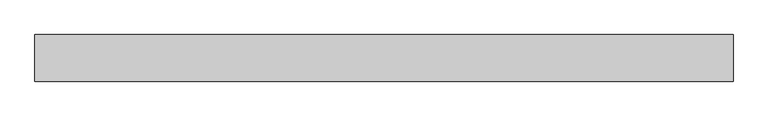
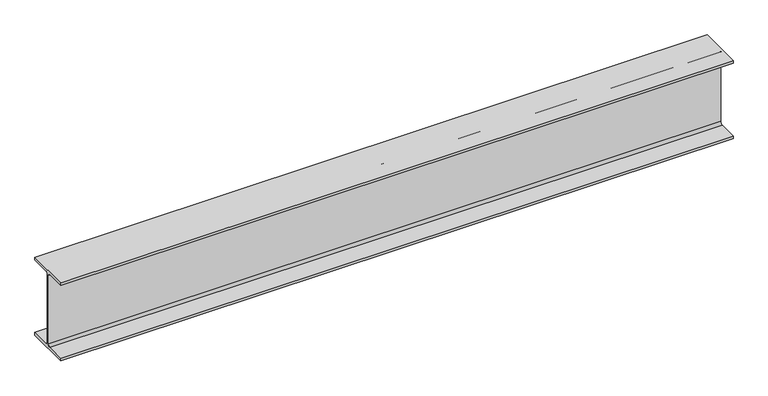
"""IFC4 building model written with IfcOpenShell, lengths in millimetres: beam geometry, Old_Steel Beam_H-KSD3502 : H_SB_ASB_H-350×175x7x11."""

from ifc_helpers import new_model, si_unit, point, frame, frame_2d, origin, place, context, project, spatial, polyline, circle_curve, trimmed, segment, composite_curve, outline, extrude, source, transform, mapped, element, save


def beam_1666eb2f(model_context):
    return source(origin(), model_context, "Body", "SweptSolid", [
        extrude(outline(composite_curve([segment(polyline([(82.5, -141.5), (82.5, -151.7), (-82.5, -151.7), (-82.5, -141.5), (-11.9, -141.5)]), True, "CONTINUOUS"), segment(trimmed(circle_curve(frame_2d((-11.9, -132.6)), 8.9), [point((-11.9, -141.5))], [point((-3.0, -132.6))], True, "CARTESIAN"), True, "CONTINUOUS"), segment(polyline([(-3.0, -132.6), (-3.0, 132.6)]), True, "CONTINUOUS"), segment(trimmed(circle_curve(frame_2d((-11.9, 132.6)), 8.9), [point((-3.0, 132.6))], [point((-11.9, 141.5))], True, "CARTESIAN"), True, "CONTINUOUS"), segment(polyline([(-11.9, 141.5), (-82.5, 141.5), (-82.5, 151.7), (82.5, 151.7), (82.5, 141.5), (11.9, 141.5)]), True, "CONTINUOUS"), segment(trimmed(circle_curve(frame_2d((11.9, 132.6)), 8.9), [point((11.9, 141.5))], [point((3.0, 132.6))], True, "CARTESIAN"), True, "CONTINUOUS"), segment(polyline([(3.0, 132.6), (3.0, -132.6)]), True, "CONTINUOUS"), segment(trimmed(circle_curve(frame_2d((11.9, -132.6)), 8.9), [point((3.0, -132.6))], [point((11.9, -141.5))], True, "CARTESIAN"), True, "CONTINUOUS"), segment(polyline([(11.9, -141.5), (82.5, -141.5)]), True, "CONTINUOUS")], self_intersect=False)), frame((-1175.6379608, 0.0, 0.0), z_axis=(1.0, 0.0, 0.0), x_axis=(0.0, 1.0, 0.0)), (0.0, 0.0, 1.0), 2471.4118659),
    ])


if __name__ == "__main__":
    model = new_model("IFC4")
    model_context = context("Model", 3, world=origin())
    ifc_project = project(units=[si_unit("LENGTHUNIT", "METRE", prefix="MILLI")], contexts=[model_context])
    site = spatial("IfcSite", under=ifc_project)
    building = spatial("IfcBuilding", under=site)
    placement = place(None, origin())
    beam_shape = beam_1666eb2f(model_context)
    element("IfcBeam", 1, ObjectType="Old_Steel Beam_H-KSD3502 : H_SB_ASB_H-350×175x7x11", at=placement, inside=building, context=model_context, shape_type="MappedRepresentation", body=[
        mapped(beam_shape, transform((0.0, 0.0, 0.0), x_axis=(1.0, 0.0, 0.0), y_axis=(0.0, 1.0, 0.0), z_axis=(0.0, 0.0, 1.0))),
    ])
    save(model, "model.ifc")

# Revit data of these elements
# Type "Old_Steel Beam_H-KSD3502 : H_SB_ASB_H-350×175x7x11"
#   Width = 17.5 cm
#   Web Thickness = 0.7 cm
#   Web Fillet = 1.4 cm
#   Warping Constant = 282290.0 cm⁶
#   Torsional Moment of Inertia = 19.4042 cm⁴
#   Torsional Modulus = 1.0 cm³
#   Section Area = 63.14 cm²
#   Plastic Modulus weak axis = 174.0 cm³
#   Plastic Modulus strong axis = 868.0 cm³
#   Perimeter = 1.36 m²/m
#   Nominal Weight = 49.60 kgf/m
#   Moment of Inertia weak axis = 984.00 cm⁴
#   Moment of Inertia strong axis = 13600.00 cm⁴
#   Height = 35.0 cm
#   Flange Thickness = 1.1 cm
#   Elastic Modulus weak axis = 112.0 cm³
#   Elastic Modulus strong axis = 775.0 cm³
#   Centroid Vertical = 17.5 cm
#   Centroid Horizontal = 8.75 cm
#   Length [instance default] = 1.5240 m
#   Structural Material [instance default] = Steel, 45-345
#   Assembly Code = ""
# Element 1 (IfcBeam, "Old_Steel Beam_H-KSD3502 : H_SB_ASB_H-350×175x7x11")
#   Structural Material = none
# Materials
#   "Steel, 45-345": class "Metal", colour RGB 189 187 185, transparency 0, Description = "Steel 345 MPa", Cost = 0
